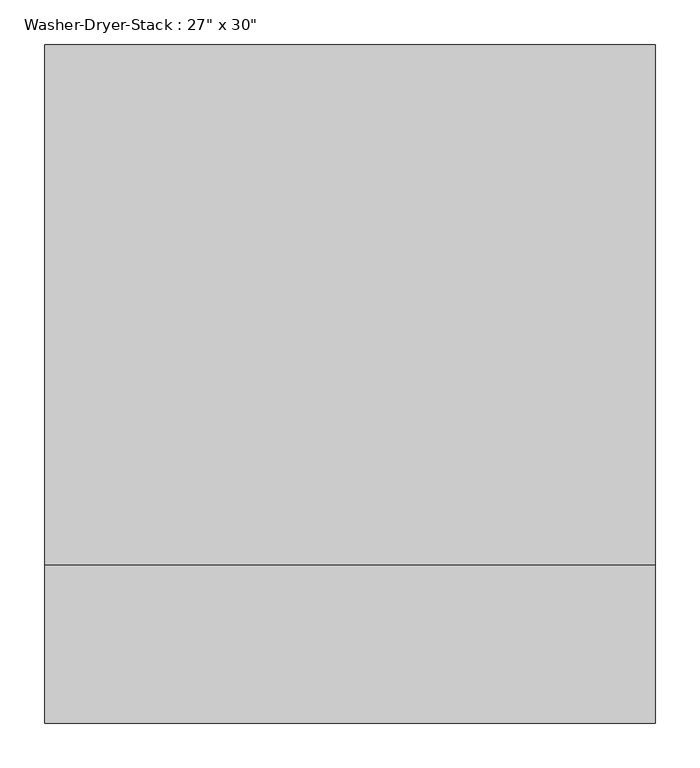
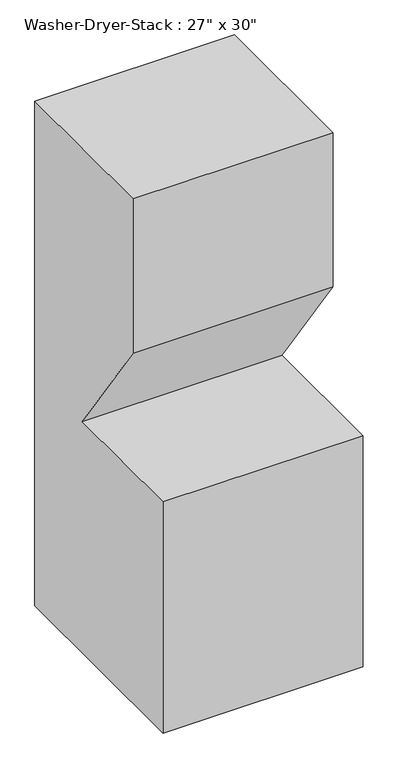
"""IFC4 building model written with IfcOpenShell, lengths in millimetres: proxy geometry."""

from ifc_helpers import new_model, si_unit, frame, origin, place, context, project, spatial, polyline, outline, extrude, source, transform, mapped, element, save


def proxy_5ec56aa7(model_context):
    return source(origin(), model_context, "Body", "SweptSolid", [
        extrude(outline(polyline([(-381.0, 0.0), (-381.0, 838.2), (99.149615, 838.2), (-203.2, 1270.0), (-203.2, 1828.8), (381.0, 1828.8), (381.0, 0.0), (-381.0, 0.0)])), frame((-342.9, 0.0, 0.0), z_axis=(1.0, 0.0, 0.0), x_axis=(0.0, 1.0, 0.0)), (0.0, 0.0, 1.0), 685.8),
    ])


if __name__ == "__main__":
    model = new_model("IFC4")
    model_context = context("Model", 3, world=origin())
    ifc_project = project(units=[si_unit("LENGTHUNIT", "METRE", prefix="MILLI")], contexts=[model_context])
    site = spatial("IfcSite", under=ifc_project)
    building = spatial("IfcBuilding", under=site)
    placement = place(None, origin())
    proxy_shape = proxy_5ec56aa7(model_context)
    element("IfcBuildingElementProxy", 1, Name="Washer-Dryer-Stack : 27\" x 30\"", ObjectType="Washer-Dryer-Stack : 27\" x 30\"", at=placement, inside=building, context=model_context, shape_type="MappedRepresentation", body=[
        mapped(proxy_shape, transform((0.0, 0.0, 0.0), x_axis=(1.0, 0.0, 0.0), y_axis=(0.0, 1.0, 0.0), z_axis=(0.0, 0.0, 1.0))),
    ])
    save(model, "model.ifc")

# Revit data of these elements
# Type "Washer-Dryer-Stack : 27\" x 30\""
#   Assembly Code = "E1090400"
#   Lower Depth = 2' - 6"
#   Upper Depth = 1' - 11"
#   Width = 2' - 3"
#   Material = Metal - Paint Finish - Ivory,Glossy
#   Default Elevation = 0
# Element 1 (IfcBuildingElementProxy, "Washer-Dryer-Stack : 27\" x 30\"")
#   Materials on its faces: "Metal - Paint Finish - Ivory,Glossy"
# Materials
#   "Metal - Paint Finish - Ivory,Glossy": class "Unassigned", colour RGB 247 247 239, transparency 0
